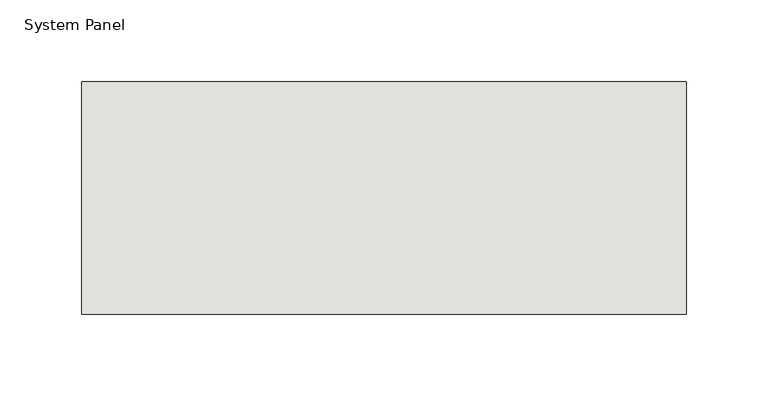
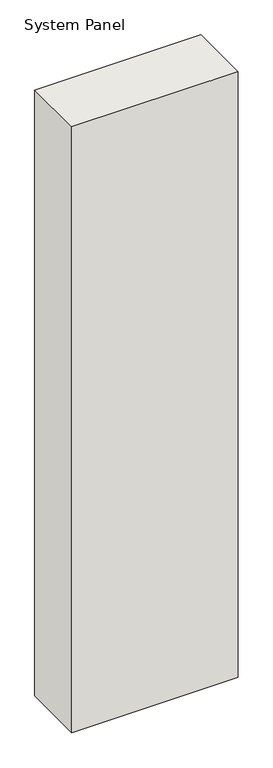
"""IFC4 building model written with IfcOpenShell, lengths in millimetres: wall geometry, System Panel : NLRS_21_CWP_hsb-vulling minerale wol 142 _gen_rsf."""

from ifc_helpers import new_model, si_unit, origin, origin_with_axes, place, context, project, spatial, polyline, outline, extrude, source, transform, mapped, element, save


def system_panel_98500bb3(model_context):
    return source(origin(), model_context, "Body", "SweptSolid", [
        extrude(outline(polyline([(184.5, -71.0), (-184.5, -71.0), (-184.5, 71.0), (184.5, 71.0), (184.5, -71.0)])), origin_with_axes(), (0.0, 0.0, 1.0), 1421.0),
    ])


if __name__ == "__main__":
    model = new_model("IFC4")
    model_context = context("Model", 3, world=origin())
    ifc_project = project(units=[si_unit("LENGTHUNIT", "METRE", prefix="MILLI")], contexts=[model_context])
    site = spatial("IfcSite", under=ifc_project)
    building = spatial("IfcBuilding", under=site)
    placement = place(None, origin())
    system_panel_shape = system_panel_98500bb3(model_context)
    element("IfcWall", 1, ObjectType="System Panel : NLRS_21_CWP_hsb-vulling minerale wol 142 _gen_rsf", at=placement, inside=building, context=model_context, shape_type="MappedRepresentation", body=[
        mapped(system_panel_shape, transform((0.0, 0.0, 0.0), x_axis=(1.0, 0.0, 0.0), y_axis=(0.0, 1.0, 0.0), z_axis=(0.0, 0.0, 1.0))),
    ])
    save(model, "model.ifc")

# Revit data of these elements
# Type "System Panel : NLRS_21_CWP_hsb-vulling minerale wol 142 _gen_rsf"
#   Type IfcGUID = "07M7mRoiH1CR8m_RSKIwpC"
#   Assembly Code = "21.23"
#   IfcExportAs = "IfcWall"
# Element 1 (IfcWall, "System Panel : NLRS_21_CWP_hsb-vulling minerale wol 142 _gen_rsf")
#   Materials on its faces: "NLRS_m1_isolatie minerale wol_gen_rsf"
# Materials
#   "NLRS_m1_isolatie minerale wol_gen_rsf": class "M - Anorganische materialen", colour RGB 200 200 140, transparency 0, Keynote = "m1", Manufacturer = "Revit Standards Foundation", URL = "www.revitstandards.org", Description = "isolatie minerale wol", Cost = 0
